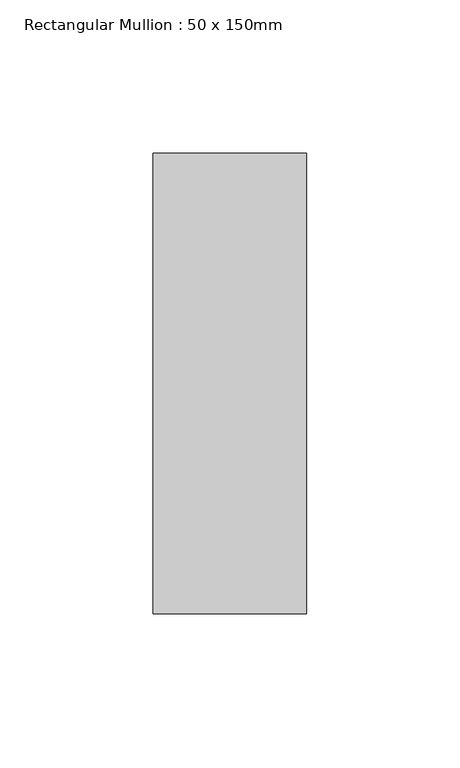
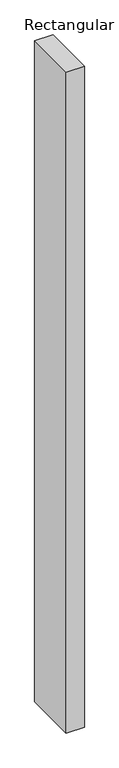
"""IFC4 building model written with IfcOpenShell, lengths in millimetres: member geometry, Rectangular Mullion : 50 x 150mm."""

from ifc_helpers import new_model, si_unit, frame, origin, place, context, project, spatial, polyline, outline, extrude, source, transform, mapped, element, save


def rectangular_mullion_50_x_150mm_7828da58(model_context):
    return source(origin(), model_context, "Body", "SweptSolid", [
        extrude(outline(polyline([(0.0, 75.0), (0.0, -75.0), (-50.0, -75.0), (-50.0, 75.0), (0.0, 75.0)])), frame((0.0, 0.0, -1923.3666669), z_axis=(0.0, 0.0, 1.0), x_axis=(1.0, 0.0, 0.0)), (0.0, 0.0, 1.0), 1923.3666669),
    ])


if __name__ == "__main__":
    model = new_model("IFC4")
    model_context = context("Model", 3, world=origin())
    ifc_project = project(units=[si_unit("LENGTHUNIT", "METRE", prefix="MILLI")], contexts=[model_context])
    site = spatial("IfcSite", under=ifc_project)
    building = spatial("IfcBuilding", under=site)
    placement = place(None, origin())
    rectangular_mullion_50_x_150mm_shape = rectangular_mullion_50_x_150mm_7828da58(model_context)
    element("IfcMember", 1, ObjectType="Rectangular Mullion : 50 x 150mm", at=placement, inside=building, context=model_context, shape_type="MappedRepresentation", body=[
        mapped(rectangular_mullion_50_x_150mm_shape, transform((0.0, 0.0, 0.0), x_axis=(1.0, 0.0, 0.0), y_axis=(0.0, 1.0, 0.0), z_axis=(0.0, 0.0, 1.0))),
    ])
    save(model, "model.ifc")

# Revit data of these elements
# Type "Rectangular Mullion : 50 x 150mm"
#   built-in parameter 1007304 = 0.492126 (stored number, unit not read)
#   built-in parameter 1007301 = 0.082021 (stored number, unit not read)
#   built-in parameter 1007300 = 0.082021 (stored number, unit not read)
# Element 1 (IfcMember, "Rectangular Mullion : 50 x 150mm")
#   Materials on its faces: "Metal - Aluminium"
# Materials
#   "Metal - Aluminium": class "Metal", colour RGB 247 247 247, transparency 0
